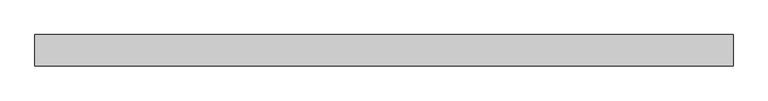
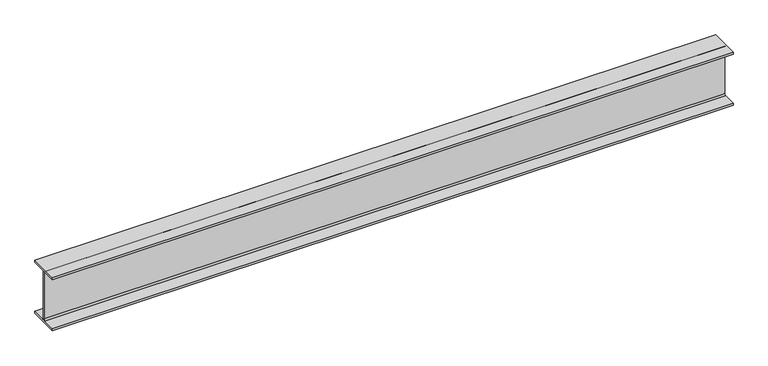
"""IFC4 building model written with IfcOpenShell, lengths in millimetres: beam geometry, Steel Beam_H-KSD3502 : H_SB_ASB_H-200x200x8x12."""

from ifc_helpers import new_model, si_unit, point, frame, frame_2d, origin, place, context, project, spatial, polyline, circle_curve, trimmed, segment, composite_curve, outline, extrude, source, transform, mapped, element, save


def beam_9a490488(model_context):
    return source(origin(), model_context, "Body", "SweptSolid", [
        extrude(outline(composite_curve([segment(polyline([(-82.5, -141.5), (-11.9, -141.5)]), True, "CONTINUOUS"), segment(trimmed(circle_curve(frame_2d((-11.9, -132.6)), 8.9), [point((-11.9, -141.5))], [point((-3.0, -132.6))], True, "CARTESIAN"), True, "CONTINUOUS"), segment(polyline([(-3.0, -132.6), (-3.0, 132.6)]), True, "CONTINUOUS"), segment(trimmed(circle_curve(frame_2d((-11.9, 132.6)), 8.9), [point((-3.0, 132.6))], [point((-11.9, 141.5))], True, "CARTESIAN"), True, "CONTINUOUS"), segment(polyline([(-11.9, 141.5), (-82.5, 141.5), (-82.5, 151.7), (82.5, 151.7), (82.5, 141.5), (11.9, 141.5)]), True, "CONTINUOUS"), segment(trimmed(circle_curve(frame_2d((11.9, 132.6)), 8.9), [point((11.9, 141.5))], [point((3.0, 132.6))], True, "CARTESIAN"), True, "CONTINUOUS"), segment(polyline([(3.0, 132.6), (3.0, -132.6)]), True, "CONTINUOUS"), segment(trimmed(circle_curve(frame_2d((11.9, -132.6)), 8.9), [point((3.0, -132.6))], [point((11.9, -141.5))], True, "CARTESIAN"), True, "CONTINUOUS"), segment(polyline([(11.9, -141.5), (82.5, -141.5), (82.5, -151.7), (-82.5, -151.7), (-82.5, -141.5)]), True, "CONTINUOUS")], self_intersect=False)), frame((-1872.8032895, 0.0, 0.0), z_axis=(1.0, 0.0, 0.0), x_axis=(0.0, 1.0, 0.0)), (0.0, 0.0, 1.0), 3693.2731785),
    ])


if __name__ == "__main__":
    model = new_model("IFC4")
    model_context = context("Model", 3, world=origin())
    ifc_project = project(units=[si_unit("LENGTHUNIT", "METRE", prefix="MILLI")], contexts=[model_context])
    site = spatial("IfcSite", under=ifc_project)
    building = spatial("IfcBuilding", under=site)
    placement = place(None, origin())
    beam_shape = beam_9a490488(model_context)
    element("IfcBeam", 1, ObjectType="Steel Beam_H-KSD3502 : H_SB_ASB_H-200x200x8x12", at=placement, inside=building, context=model_context, shape_type="MappedRepresentation", body=[
        mapped(beam_shape, transform((0.0, 0.0, 0.0), x_axis=(1.0, 0.0, 0.0), y_axis=(0.0, 1.0, 0.0), z_axis=(0.0, 0.0, 1.0))),
    ])
    save(model, "model.ifc")

# Revit data of these elements
# Type "Steel Beam_H-KSD3502 : H_SB_ASB_H-200x200x8x12"
#   Width = 20.0 cm
#   Web Thickness = 0.8 cm
#   Web Fillet = 1.3 cm
#   Warping Constant = 141376.0 cm⁶
#   Torsional Moment of Inertia = 26.2485 cm⁴
#   Torsional Modulus = 1.0 cm³
#   Section Area = 63.53 cm²
#   Plastic Modulus weak axis = 244.0 cm³
#   Plastic Modulus strong axis = 525.0 cm³
#   Perimeter = 1.16 m²/m
#   Nominal Weight = 49.90 kgf/m
#   Moment of Inertia weak axis = 1600.00 cm⁴
#   Moment of Inertia strong axis = 4720.00 cm⁴
#   Height = 20.0 cm
#   Flange Thickness = 1.2 cm
#   Elastic Modulus weak axis = 160.0 cm³
#   Elastic Modulus strong axis = 472.0 cm³
#   Centroid Vertical = 10.0 cm
#   Centroid Horizontal = 10.0 cm
#   Length [instance default] = 1.5240 m
#   Structural Material [instance default] = Steel, 45-345
#   Assembly Code = ""
# Element 1 (IfcBeam, "Steel Beam_H-KSD3502 : H_SB_ASB_H-200x200x8x12")
#   Structural Material = none
# Materials
#   "Steel, 45-345": class "Metal", colour RGB 189 187 185, transparency 0, Description = "Steel 345 MPa", Cost = 0
